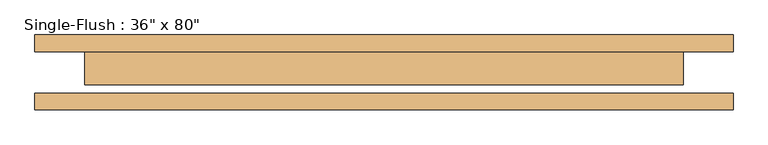
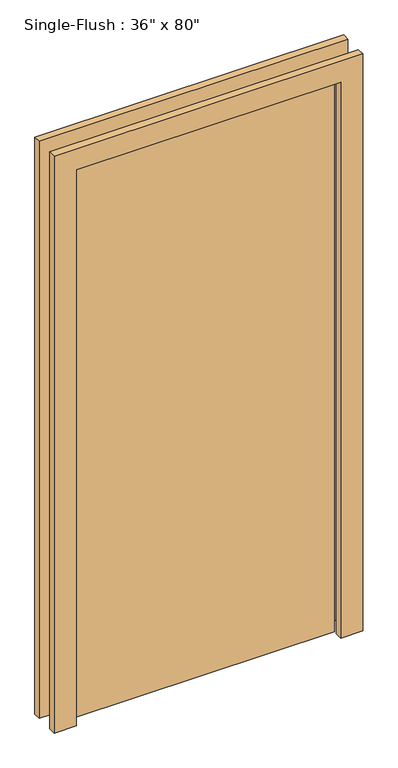
"""IFC4 building model written with IfcOpenShell, lengths in millimetres: door geometry."""

import ifcopenshell
import ifcopenshell.guid

model = None  # the IFC model being written
_history = None  # IfcOwnerHistory: only IFC2X3 demands one
_inside = {}  # id of a spatial element -> (the spatial element, [elements in it])
_under = {}  # id of a project, library or spatial element -> (it, [spatial elements below it])
_declared = {}  # id of a project -> (the project, [libraries it declares])
_typed = {}  # id of a type object -> (the type object, [elements of that type])
_made_of = {}  # id of a material, layer set ... -> (it, [elements and type objects made of it])


def new_model(schema):
    """Start an empty IFC model of exactly this schema.

    Asked for "IFC4X3", IfcOpenShell would pick the latest addendum, in which some entities
    have other attributes; the version numbers below select the first issue.
    IFC2X3 requires an IfcOwnerHistory on every rooted entity: one is made here for all.
    """
    global model, _history
    if schema == "IFC4X3":
        model = ifcopenshell.file(schema_version=(4, 3, 0, 0))
    else:
        model = ifcopenshell.file(schema=schema)
    _inside.clear()
    _under.clear()
    _declared.clear()
    _typed.clear()
    _made_of.clear()
    _history = None
    if model.schema == "IFC2X3":
        org = make("IfcOrganization", Name="unknown")
        user = make(
            "IfcPersonAndOrganization",
            ThePerson=make("IfcPerson", FamilyName="unknown"),
            TheOrganization=org,
        )
        app = make(
            "IfcApplication",
            ApplicationDeveloper=org,
            Version="unknown",
            ApplicationFullName="unknown",
            ApplicationIdentifier="unknown",
        )
        _history = make(
            "IfcOwnerHistory",
            OwningUser=user,
            OwningApplication=app,
            ChangeAction="ADDED",
            CreationDate=0,
        )
    return model


def make(cls, **values):
    """One entity of the class cls with the attributes given. An attribute that is None is left unset."""
    return model.create_entity(
        cls, **{name: value for name, value in values.items() if value is not None}
    )


def rooted(cls, **values):
    """An entity with a GlobalId (a new one), such as an element, a storey or a relation."""
    return make(cls, GlobalId=ifcopenshell.guid.new(), OwnerHistory=_history, **values)


def si_unit(unit_type, name, prefix=None):
    """IfcSIUnit, for example si_unit("LENGTHUNIT", "METRE", prefix="MILLI")."""
    return make("IfcSIUnit", UnitType=unit_type, Prefix=prefix, Name=name)


def assignment(units):
    """IfcUnitAssignment: the units of a project."""
    return None if units is None else make("IfcUnitAssignment", Units=units)


def point(xyz):
    """IfcCartesianPoint."""
    return None if xyz is None else make("IfcCartesianPoint", Coordinates=xyz)


def direction(xyz):
    """IfcDirection."""
    return None if xyz is None else make("IfcDirection", DirectionRatios=xyz)


def frame(location, z_axis=None, x_axis=None):
    """IfcAxis2Placement3D, a coordinate frame: its origin and axes. An axis left out is left unset."""
    return make(
        "IfcAxis2Placement3D",
        Location=point(location),
        Axis=direction(z_axis),
        RefDirection=direction(x_axis),
    )


def origin():
    """The frame at (0, 0, 0) with its axes left unset."""
    return frame((0.0, 0.0, 0.0))


def origin_with_axes():
    """The frame at (0, 0, 0) with the z axis (0, 0, 1) and the x axis (1, 0, 0) written out."""
    return frame((0.0, 0.0, 0.0), z_axis=(0.0, 0.0, 1.0), x_axis=(1.0, 0.0, 0.0))


def place(relative_to, where):
    """IfcLocalPlacement: puts the frame where relative to a parent placement (None: the world)."""
    return make(
        "IfcLocalPlacement", PlacementRelTo=relative_to, RelativePlacement=where
    )


def context(
    kind, dimensions, precision=None, world=None, true_north=None, identifier=None
):
    """IfcGeometricRepresentationContext, for example the 3D "Model" context."""
    return make(
        "IfcGeometricRepresentationContext",
        ContextIdentifier=identifier,
        ContextType=kind,
        CoordinateSpaceDimension=dimensions,
        Precision=precision,
        WorldCoordinateSystem=world,
        TrueNorth=true_north,
    )


def project(units=None, contexts=None):
    """IfcProject with its units and contexts."""
    return rooted(
        "IfcProject",
        Name="project",
        RepresentationContexts=contexts,
        UnitsInContext=assignment(units),
    )


def spatial(cls, under=None, at=None, **own):
    """A site, building, storey or space (cls), placed at a placement, below another one or the project."""
    s = rooted(cls, ObjectPlacement=at, **own)
    if under is not None:
        _under.setdefault(under.id(), (under, []))[1].append(s)
    return s


def polyline(points):
    """IfcPolyline through the points."""
    return make("IfcPolyline", Points=[point(p) for p in points])


def outline(outer, holes=None, kind="AREA"):
    """IfcArbitraryClosedProfileDef: a profile drawn as a closed curve; with holes, ...WithVoids."""
    if holes is None:
        return make("IfcArbitraryClosedProfileDef", ProfileType=kind, OuterCurve=outer)
    return make(
        "IfcArbitraryProfileDefWithVoids",
        ProfileType=kind,
        OuterCurve=outer,
        InnerCurves=holes,
    )


def extrude(swept, where, along, depth):
    """IfcExtrudedAreaSolid: the profile swept, set in the frame where, extruded along a direction by depth."""
    return make(
        "IfcExtrudedAreaSolid",
        SweptArea=swept,
        Position=where,
        ExtrudedDirection=direction(along),
        Depth=depth,
    )


def shape(context_of_items, identifier, shape_type, items):
    """IfcShapeRepresentation: the items that make up one representation, for example the "Body"."""
    return make(
        "IfcShapeRepresentation",
        ContextOfItems=context_of_items,
        RepresentationIdentifier=identifier,
        RepresentationType=shape_type,
        Items=items,
    )


def source(mapping_origin, context_of_items, identifier, shape_type, items):
    """IfcRepresentationMap: a shape defined once, which mapped items show again and again."""
    return make(
        "IfcRepresentationMap",
        MappingOrigin=mapping_origin,
        MappedRepresentation=shape(context_of_items, identifier, shape_type, items),
    )


def transform(
    local_origin,
    x_axis=None,
    y_axis=None,
    z_axis=None,
    scale=None,
    scale2=None,
    scale3=None,
    uniform=True,
):
    """IfcCartesianTransformationOperator3D, or its non-uniform kind. x_axis, y_axis, z_axis: its Axis1, 2, 3."""
    if uniform:
        return make(
            "IfcCartesianTransformationOperator3D",
            Axis1=direction(x_axis),
            Axis2=direction(y_axis),
            LocalOrigin=point(local_origin),
            Scale=scale,
            Axis3=direction(z_axis),
        )
    return make(
        "IfcCartesianTransformationOperator3DnonUniform",
        Axis1=direction(x_axis),
        Axis2=direction(y_axis),
        LocalOrigin=point(local_origin),
        Scale=scale,
        Axis3=direction(z_axis),
        Scale2=scale2,
        Scale3=scale3,
    )


def mapped(mapping_source, mapping_target):
    """IfcMappedItem: shows the shape of a source again, moved by a transform."""
    return make(
        "IfcMappedItem", MappingSource=mapping_source, MappingTarget=mapping_target
    )


def made_of(thing, what):
    """Note that an element or type object is made of a material, layer set ...; save() writes the relation."""
    if what is not None:
        _made_of.setdefault(what.id(), (what, []))[1].append(thing)
    return thing


def element(
    cls,
    number,
    at=None,
    inside=None,
    cuts=None,
    type_object=None,
    material=None,
    context=None,
    identifier="Body",
    shape_type=None,
    held_by="IfcProductDefinitionShape",
    body=None,
    shapes=None,
    **own,
):
    """One element of the class cls, such as IfcWall. Its Tag is "e" and its number.

    at: its placement. inside: the storey or other place that contains it. cuts: it is an
    opening in that element (IfcRelVoidsElement). A single representation is given by context,
    identifier, shape_type and body (its items); several are given by shapes. held_by: the class
    of the entity that holds the representations. save() writes the other relations.
    """
    e = rooted(cls, Tag="e%d" % number, ObjectPlacement=at, **own)
    if body is not None:
        shapes = [shape(context, identifier, shape_type, body)]
    if shapes is not None:
        e.Representation = make(held_by, Representations=shapes)
    if inside is not None:
        _inside.setdefault(inside.id(), (inside, []))[1].append(e)
    if cuts is not None:
        rooted(
            "IfcRelVoidsElement", RelatingBuildingElement=cuts, RelatedOpeningElement=e
        )
    if type_object is not None:
        _typed.setdefault(type_object.id(), (type_object, []))[1].append(e)
    return made_of(e, material)


def aggregate(whole, parts):
    """IfcRelAggregates: a whole, such as a stair, and the parts it consists of."""
    return rooted("IfcRelAggregates", RelatingObject=whole, RelatedObjects=parts)


def save(model, path):
    """Write the relations noted so far, then the file.

    IfcRelAggregates (storeys below a building ...), IfcRelContainedInSpatialStructure (elements
    in a storey), IfcRelDefinesByType, IfcRelAssociatesMaterial and IfcRelDeclares: one each for
    every whole, place, type object, material and project.
    """
    for whole, parts in _under.values():
        aggregate(whole, parts)
    for where, things in _inside.values():
        rooted(
            "IfcRelContainedInSpatialStructure",
            RelatedElements=things,
            RelatingStructure=where,
        )
    for kind, things in _typed.values():
        rooted("IfcRelDefinesByType", RelatedObjects=things, RelatingType=kind)
    for what, things in _made_of.values():
        rooted("IfcRelAssociatesMaterial", RelatedObjects=things, RelatingMaterial=what)
    for by, libraries in _declared.values():
        rooted("IfcRelDeclares", RelatingContext=by, RelatedDefinitions=libraries)
    model.write(path)


def door_67b2d19c(model_context):
    return source(origin(), model_context, "Body", "SweptSolid", [
        extrude(outline(polyline([(2108.2, -533.4), (0.0, -533.4), (0.0, -457.2), (2032.0, -457.2), (2032.0, 457.2), (0.0, 457.2), (0.0, 533.4), (2108.2, 533.4), (2108.2, -533.4)])), frame((0.0, 31.75, 0.0), z_axis=(0.0, 1.0, 0.0), x_axis=(0.0, 0.0, 1.0)), (0.0, 0.0, 1.0), 25.4),
        extrude(outline(polyline([(2108.2, 533.4), (2108.2, -533.4), (0.0, -533.4), (0.0, -457.2), (2032.0, -457.2), (2032.0, 457.2), (0.0, 457.2), (0.0, 533.4), (2108.2, 533.4)])), frame((0.0, -57.15, 0.0), z_axis=(0.0, 1.0, 0.0), x_axis=(0.0, 0.0, 1.0)), (0.0, 0.0, 1.0), 25.4),
        extrude(outline(polyline([(457.2, -19.05), (-457.2, -19.05), (-457.2, 31.75), (457.2, 31.75), (457.2, -19.05)])), origin_with_axes(), (0.0, 0.0, 1.0), 2032.0),
    ])


if __name__ == "__main__":
    model = new_model("IFC4")
    model_context = context("Model", 3, world=origin())
    ifc_project = project(units=[si_unit("LENGTHUNIT", "METRE", prefix="MILLI")], contexts=[model_context])
    site = spatial("IfcSite", under=ifc_project)
    building = spatial("IfcBuilding", under=site)
    placement = place(None, origin())
    door_shape = door_67b2d19c(model_context)
    element("IfcDoor", 1, ObjectType="Single-Flush : 36\" x 80\"", at=placement, inside=building, context=model_context, shape_type="MappedRepresentation", body=[
        mapped(door_shape, transform((0.0, 0.0, 0.0), x_axis=(1.0, 0.0, 0.0), y_axis=(0.0, 1.0, 0.0), z_axis=(0.0, 0.0, 1.0))),
    ])
    save(model, "model.ifc")

# Revit data of these elements
# Type "Single-Flush : 36\" x 80\""
#   Type Mark = "6"
#   Construction Type Id = "MDOOR"
#   Assembly Code = "C1020"
#   Analytic Construction = "Metal"
#   Thickness = 0' - 2"
#   Heat Transfer Coefficient (U) = 0.651978 BTU/(h·ft²·°F)
#   Height = 6' - 8"
#   Trim Projection Ext = 0' - 1"
#   Trim Projection Int = 0' - 1"
#   Trim Width = 0' - 3"
#   Width = 3' - 0"
#   Define Thermal Properties by = 1
#   Define Thermal Properties by = 1
#   Door Material = Door - Panel
#   Frame Material = Door - Frame
#   Visual Light Transmittance = 0
#   Solar Heat Gain Coefficient = 0
#   Function = (empty or 0)
#   Wall Closure = (empty or 0)
# Element 1 (IfcDoor, "Single-Flush : 36\" x 80\"")
#   Materials on its faces: "Door - Frame", "Door - Panel"
# Materials
#   "Door - Panel": class "Wood", colour RGB 210 159 95, transparency 0, Cost = 0
#   "Door - Frame": class "Miscellaneous", colour RGB 118 70 51, transparency 0, Cost = 0
